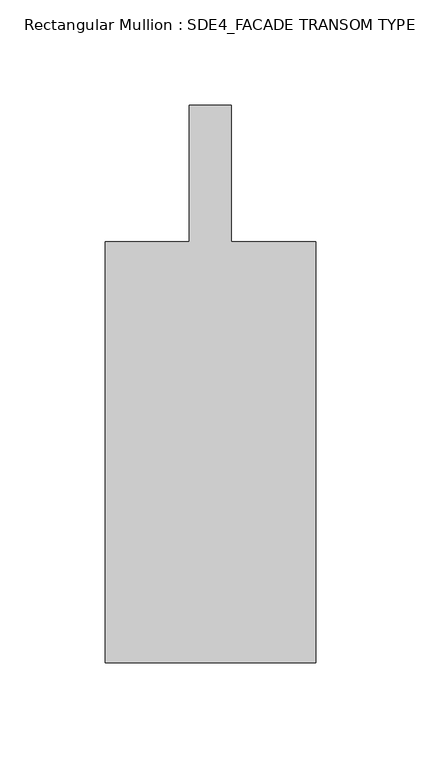
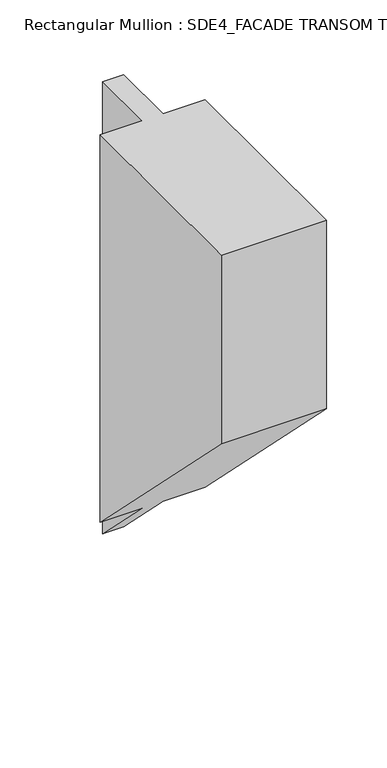
"""IFC4 building model written with IfcOpenShell, lengths in millimetres: member geometry, Rectangular Mullion : SDE4_FACADE TRANSOM TYPE 2."""

from ifc_helpers import new_model, si_unit, origin, place, context, project, spatial, faceted_brep, source, transform, mapped, element, save


def rectangular_mullion_sde4_facade_transom_type_2_43e1a6bb(model_context):
    return source(origin(), model_context, "Body", "Brep", [
        faceted_brep([(50.0, -132.5, 0.0), (50.0, 67.5, 0.0), (10.0, 67.5, 0.0), (10.0, 132.5, 0.0), (-10.0, 132.5, 0.0), (-10.0, 67.5, 0.0), (-50.0, 67.5, 0.0), (-50.0, -132.5, 0.0), (50.0, -132.5, -189.5970392), (50.0, 67.5, -389.5970392), (10.0, 67.5, -389.5970392), (10.0, 132.5, -454.5970392), (-10.0, 132.5, -454.5970392), (-10.0, 67.5, -389.5970392), (-50.0, 67.5, -389.5970392), (-50.0, -132.5, -189.5970392)], [[[0, 1, 2, 3, 4, 5, 6, 7]], [[1, 0, 8, 9]], [[2, 1, 9, 10]], [[3, 2, 10, 11]], [[4, 3, 11, 12]], [[5, 4, 12, 13]], [[6, 5, 13, 14]], [[7, 6, 14, 15]], [[0, 7, 15, 8]], [[8, 15, 14, 13, 12, 11, 10, 9]]]),
    ])


if __name__ == "__main__":
    model = new_model("IFC4")
    model_context = context("Model", 3, world=origin())
    ifc_project = project(units=[si_unit("LENGTHUNIT", "METRE", prefix="MILLI")], contexts=[model_context])
    site = spatial("IfcSite", under=ifc_project)
    building = spatial("IfcBuilding", under=site)
    placement = place(None, origin())
    rectangular_mullion_sde4_facade_transom_type_2_shape = rectangular_mullion_sde4_facade_transom_type_2_43e1a6bb(model_context)
    element("IfcMember", 1, ObjectType="Rectangular Mullion : SDE4_FACADE TRANSOM TYPE 2", at=placement, inside=building, context=model_context, shape_type="MappedRepresentation", body=[
        mapped(rectangular_mullion_sde4_facade_transom_type_2_shape, transform((0.0, 0.0, 0.0), x_axis=(1.0, 0.0, 0.0), y_axis=(0.0, 1.0, 0.0), z_axis=(0.0, 0.0, 1.0))),
    ])
    save(model, "model.ifc")

# Revit data of these elements
# Type "Rectangular Mullion : SDE4_FACADE TRANSOM TYPE 2"
#   built-in parameter 1007322 = 0.869423 (stored number, unit not read)
#   built-in parameter 1007321 = 0.164042 (stored number, unit not read)
#   built-in parameter 1007320 = 0.164042 (stored number, unit not read)
